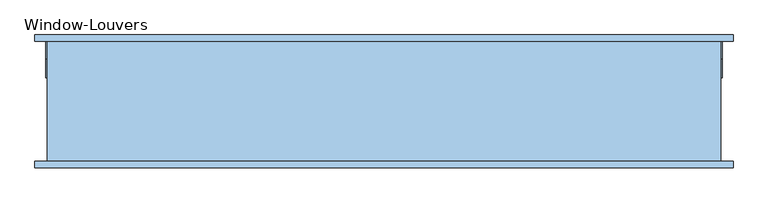
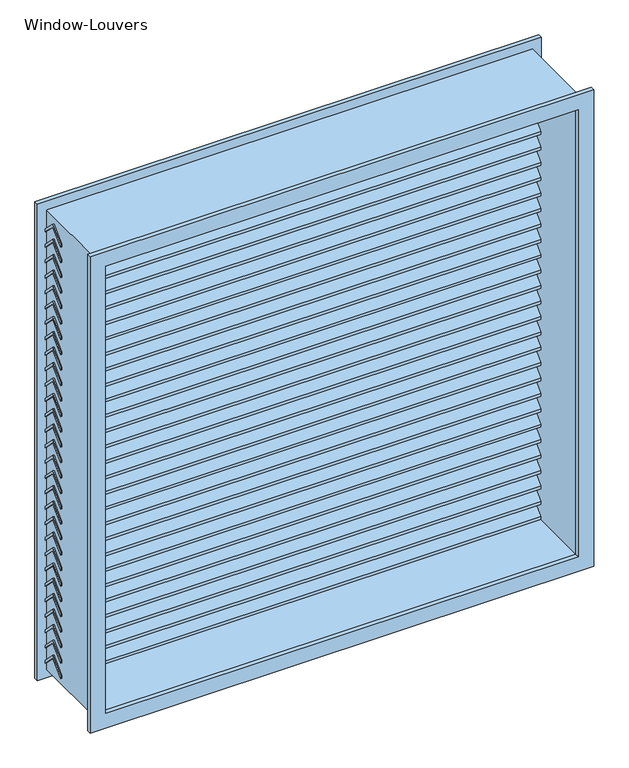
"""IFC4 building model written with IfcOpenShell, lengths in millimetres: window geometry, Window-Louvers : H_WD_AR_B11_Louver_Steel_W1450xH1450."""

from ifc_helpers import new_model, si_unit, frame, origin, place, context, project, spatial, polyline, outline, extrude, source, transform, mapped, element, save


def window_louvers_5883d314(model_context):
    return source(origin(), model_context, "Body", "SweptSolid", [
        extrude(outline(polyline([(118.65, 2234.4100091), (118.65, 2225.429753), (80.55, 2263.529753), (42.45, 2225.429753), (42.45, 2234.4100091), (80.55, 2272.5100091), (118.65, 2234.4100091)])), frame((-702.5, 0.0, 0.0), z_axis=(1.0, 0.0, 0.0), x_axis=(0.0, 1.0, 0.0)), (0.0, 0.0, 1.0), 1405.0),
        extrude(outline(polyline([(118.65, 2187.5200183), (118.65, 2178.5397622), (80.55, 2216.6397622), (42.45, 2178.5397622), (42.45, 2187.5200183), (80.55, 2225.6200183), (118.65, 2187.5200183)])), frame((-702.5, 0.0, 0.0), z_axis=(1.0, 0.0, 0.0), x_axis=(0.0, 1.0, 0.0)), (0.0, 0.0, 1.0), 1405.0),
        extrude(outline(polyline([(118.65, 2140.6300274), (118.65, 2131.6497713), (80.55, 2169.7497713), (42.45, 2131.6497713), (42.45, 2140.6300274), (80.55, 2178.7300274), (118.65, 2140.6300274)])), frame((-702.5, 0.0, 0.0), z_axis=(1.0, 0.0, 0.0), x_axis=(0.0, 1.0, 0.0)), (0.0, 0.0, 1.0), 1405.0),
        extrude(outline(polyline([(118.65, 2093.7400366), (118.65, 2084.7597805), (80.55, 2122.8597805), (42.45, 2084.7597805), (42.45, 2093.7400366), (80.55, 2131.8400366), (118.65, 2093.7400366)])), frame((-702.5, 0.0, 0.0), z_axis=(1.0, 0.0, 0.0), x_axis=(0.0, 1.0, 0.0)), (0.0, 0.0, 1.0), 1405.0),
        extrude(outline(polyline([(118.65, 2046.8500457), (118.65, 2037.8697896), (80.55, 2075.9697896), (42.45, 2037.8697896), (42.45, 2046.8500457), (80.55, 2084.9500457), (118.65, 2046.8500457)])), frame((-702.5, 0.0, 0.0), z_axis=(1.0, 0.0, 0.0), x_axis=(0.0, 1.0, 0.0)), (0.0, 0.0, 1.0), 1405.0),
        extrude(outline(polyline([(118.65, 1999.9600549), (118.65, 1990.9797988), (80.55, 2029.0797988), (42.45, 1990.9797988), (42.45, 1999.9600549), (80.55, 2038.0600549), (118.65, 1999.9600549)])), frame((-702.5, 0.0, 0.0), z_axis=(1.0, 0.0, 0.0), x_axis=(0.0, 1.0, 0.0)), (0.0, 0.0, 1.0), 1405.0),
        extrude(outline(polyline([(118.65, 1953.070064), (118.65, 1944.0898079), (80.55, 1982.1898079), (42.45, 1944.0898079), (42.45, 1953.070064), (80.55, 1991.170064), (118.65, 1953.070064)])), frame((-702.5, 0.0, 0.0), z_axis=(1.0, 0.0, 0.0), x_axis=(0.0, 1.0, 0.0)), (0.0, 0.0, 1.0), 1405.0),
        extrude(outline(polyline([(118.65, 1906.1800732), (118.65, 1897.1998171), (80.55, 1935.2998171), (42.45, 1897.1998171), (42.45, 1906.1800732), (80.55, 1944.2800732), (118.65, 1906.1800732)])), frame((-702.5, 0.0, 0.0), z_axis=(1.0, 0.0, 0.0), x_axis=(0.0, 1.0, 0.0)), (0.0, 0.0, 1.0), 1405.0),
        extrude(outline(polyline([(118.65, 1859.2900823), (118.65, 1850.3098262), (80.55, 1888.4098262), (42.45, 1850.3098262), (42.45, 1859.2900823), (80.55, 1897.3900823), (118.65, 1859.2900823)])), frame((-702.5, 0.0, 0.0), z_axis=(1.0, 0.0, 0.0), x_axis=(0.0, 1.0, 0.0)), (0.0, 0.0, 1.0), 1405.0),
        extrude(outline(polyline([(118.65, 1812.4000915), (118.65, 1803.4198354), (80.55, 1841.5198354), (42.45, 1803.4198354), (42.45, 1812.4000915), (80.55, 1850.5000915), (118.65, 1812.4000915)])), frame((-702.5, 0.0, 0.0), z_axis=(1.0, 0.0, 0.0), x_axis=(0.0, 1.0, 0.0)), (0.0, 0.0, 1.0), 1405.0),
        extrude(outline(polyline([(118.65, 1765.5101006), (118.65, 1756.5298445), (80.55, 1794.6298445), (42.45, 1756.5298445), (42.45, 1765.5101006), (80.55, 1803.6101006), (118.65, 1765.5101006)])), frame((-702.5, 0.0, 0.0), z_axis=(1.0, 0.0, 0.0), x_axis=(0.0, 1.0, 0.0)), (0.0, 0.0, 1.0), 1405.0),
        extrude(outline(polyline([(118.65, 1718.6201098), (118.65, 1709.6398536), (80.55, 1747.7398536), (42.45, 1709.6398536), (42.45, 1718.6201098), (80.55, 1756.7201098), (118.65, 1718.6201098)])), frame((-702.5, 0.0, 0.0), z_axis=(1.0, 0.0, 0.0), x_axis=(0.0, 1.0, 0.0)), (0.0, 0.0, 1.0), 1405.0),
        extrude(outline(polyline([(118.65, 1671.7301189), (118.65, 1662.7498628), (80.55, 1700.8498628), (42.45, 1662.7498628), (42.45, 1671.7301189), (80.55, 1709.8301189), (118.65, 1671.7301189)])), frame((-702.5, 0.0, 0.0), z_axis=(1.0, 0.0, 0.0), x_axis=(0.0, 1.0, 0.0)), (0.0, 0.0, 1.0), 1405.0),
        extrude(outline(polyline([(118.65, 1624.8401281), (118.65, 1615.8598719), (80.55, 1653.9598719), (42.45, 1615.8598719), (42.45, 1624.8401281), (80.55, 1662.9401281), (118.65, 1624.8401281)])), frame((-702.5, 0.0, 0.0), z_axis=(1.0, 0.0, 0.0), x_axis=(0.0, 1.0, 0.0)), (0.0, 0.0, 1.0), 1405.0),
        extrude(outline(polyline([(118.65, 1577.9501372), (118.65, 1568.9698811), (80.55, 1607.0698811), (42.45, 1568.9698811), (42.45, 1577.9501372), (80.55, 1616.0501372), (118.65, 1577.9501372)])), frame((-702.5, 0.0, 0.0), z_axis=(1.0, 0.0, 0.0), x_axis=(0.0, 1.0, 0.0)), (0.0, 0.0, 1.0), 1405.0),
        extrude(outline(polyline([(118.65, 1531.0601464), (118.65, 1522.0798902), (80.55, 1560.1798902), (42.45, 1522.0798902), (42.45, 1531.0601464), (80.55, 1569.1601464), (118.65, 1531.0601464)])), frame((-702.5, 0.0, 0.0), z_axis=(1.0, 0.0, 0.0), x_axis=(0.0, 1.0, 0.0)), (0.0, 0.0, 1.0), 1405.0),
        extrude(outline(polyline([(118.65, 1484.1701555), (118.65, 1475.1898994), (80.55, 1513.2898994), (42.45, 1475.1898994), (42.45, 1484.1701555), (80.55, 1522.2701555), (118.65, 1484.1701555)])), frame((-702.5, 0.0, 0.0), z_axis=(1.0, 0.0, 0.0), x_axis=(0.0, 1.0, 0.0)), (0.0, 0.0, 1.0), 1405.0),
        extrude(outline(polyline([(118.65, 1437.2801646), (118.65, 1428.2999085), (80.55, 1466.3999085), (42.45, 1428.2999085), (42.45, 1437.2801646), (80.55, 1475.3801646), (118.65, 1437.2801646)])), frame((-702.5, 0.0, 0.0), z_axis=(1.0, 0.0, 0.0), x_axis=(0.0, 1.0, 0.0)), (0.0, 0.0, 1.0), 1405.0),
        extrude(outline(polyline([(118.65, 1390.3901738), (118.65, 1381.4099177), (80.55, 1419.5099177), (42.45, 1381.4099177), (42.45, 1390.3901738), (80.55, 1428.4901738), (118.65, 1390.3901738)])), frame((-702.5, 0.0, 0.0), z_axis=(1.0, 0.0, 0.0), x_axis=(0.0, 1.0, 0.0)), (0.0, 0.0, 1.0), 1405.0),
        extrude(outline(polyline([(118.65, 1343.5001829), (118.65, 1334.5199268), (80.55, 1372.6199268), (42.45, 1334.5199268), (42.45, 1343.5001829), (80.55, 1381.6001829), (118.65, 1343.5001829)])), frame((-702.5, 0.0, 0.0), z_axis=(1.0, 0.0, 0.0), x_axis=(0.0, 1.0, 0.0)), (0.0, 0.0, 1.0), 1405.0),
        extrude(outline(polyline([(118.65, 1296.6101921), (118.65, 1287.629936), (80.55, 1325.729936), (42.45, 1287.629936), (42.45, 1296.6101921), (80.55, 1334.7101921), (118.65, 1296.6101921)])), frame((-702.5, 0.0, 0.0), z_axis=(1.0, 0.0, 0.0), x_axis=(0.0, 1.0, 0.0)), (0.0, 0.0, 1.0), 1405.0),
        extrude(outline(polyline([(118.65, 1249.7202012), (118.65, 1240.7399451), (80.55, 1278.8399451), (42.45, 1240.7399451), (42.45, 1249.7202012), (80.55, 1287.8202012), (118.65, 1249.7202012)])), frame((-702.5, 0.0, 0.0), z_axis=(1.0, 0.0, 0.0), x_axis=(0.0, 1.0, 0.0)), (0.0, 0.0, 1.0), 1405.0),
        extrude(outline(polyline([(118.65, 1202.8302104), (118.65, 1193.8499543), (80.55, 1231.9499543), (42.45, 1193.8499543), (42.45, 1202.8302104), (80.55, 1240.9302104), (118.65, 1202.8302104)])), frame((-702.5, 0.0, 0.0), z_axis=(1.0, 0.0, 0.0), x_axis=(0.0, 1.0, 0.0)), (0.0, 0.0, 1.0), 1405.0),
        extrude(outline(polyline([(118.65, 1155.9402195), (118.65, 1146.9599634), (80.55, 1185.0599634), (42.45, 1146.9599634), (42.45, 1155.9402195), (80.55, 1194.0402195), (118.65, 1155.9402195)])), frame((-702.5, 0.0, 0.0), z_axis=(1.0, 0.0, 0.0), x_axis=(0.0, 1.0, 0.0)), (0.0, 0.0, 1.0), 1405.0),
        extrude(outline(polyline([(118.65, 1109.0502287), (118.65, 1100.0699726), (80.55, 1138.1699726), (42.45, 1100.0699726), (42.45, 1109.0502287), (80.55, 1147.1502287), (118.65, 1109.0502287)])), frame((-702.5, 0.0, 0.0), z_axis=(1.0, 0.0, 0.0), x_axis=(0.0, 1.0, 0.0)), (0.0, 0.0, 1.0), 1405.0),
        extrude(outline(polyline([(118.65, 1062.1602378), (118.65, 1053.1799817), (80.55, 1091.2799817), (42.45, 1053.1799817), (42.45, 1062.1602378), (80.55, 1100.2602378), (118.65, 1062.1602378)])), frame((-702.5, 0.0, 0.0), z_axis=(1.0, 0.0, 0.0), x_axis=(0.0, 1.0, 0.0)), (0.0, 0.0, 1.0), 1405.0),
        extrude(outline(polyline([(118.65, 1015.270247), (118.65, 1006.2899909), (80.55, 1044.3899909), (42.45, 1006.2899909), (42.45, 1015.270247), (80.55, 1053.370247), (118.65, 1015.270247)])), frame((-702.5, 0.0, 0.0), z_axis=(1.0, 0.0, 0.0), x_axis=(0.0, 1.0, 0.0)), (0.0, 0.0, 1.0), 1405.0),
        extrude(outline(polyline([(118.65, 2281.3), (118.65, 2272.3197439), (80.55, 2310.4197439), (42.45, 2272.3197439), (42.45, 2281.3), (80.55, 2319.4), (118.65, 2281.3)])), frame((-702.5, 0.0, 0.0), z_axis=(1.0, 0.0, 0.0), x_axis=(0.0, 1.0, 0.0)), (0.0, 0.0, 1.0), 1405.0),
        extrude(outline(polyline([(118.65, 968.3802561), (118.65, 959.4), (80.55, 997.5), (42.45, 959.4), (42.45, 968.3802561), (80.55, 1006.4802561), (118.65, 968.3802561)])), frame((-702.5, 0.0, 0.0), z_axis=(1.0, 0.0, 0.0), x_axis=(0.0, 1.0, 0.0)), (0.0, 0.0, 1.0), 1405.0),
        extrude(outline(polyline([(2364.4, -725.0), (914.4, -725.0), (914.4, 725.0), (2364.4, 725.0), (2364.4, -725.0)]), holes=[polyline([(2319.4, -680.0), (2319.4, 680.0), (959.4, 680.0), (959.4, -680.0), (2319.4, -680.0)])]), frame((0.0, 118.65, 0.0), z_axis=(0.0, 1.0, 0.0), x_axis=(0.0, 0.0, 1.0)), (0.0, 0.0, 1.0), 12.7),
        extrude(outline(polyline([(2364.4, 725.0), (2364.4, -725.0), (914.4, -725.0), (914.4, 725.0), (2364.4, 725.0)]), holes=[polyline([(2319.4, 680.0), (959.4, 680.0), (959.4, -680.0), (2319.4, -680.0), (2319.4, 680.0)])]), frame((0.0, -144.05, 0.0), z_axis=(0.0, 1.0, 0.0), x_axis=(0.0, 0.0, 1.0)), (0.0, 0.0, 1.0), 12.7),
        extrude(outline(polyline([(2338.45, 699.05), (2338.45, -699.05), (940.35, -699.05), (940.35, 699.05), (2338.45, 699.05)]), holes=[polyline([(2319.4, 680.0), (959.4, 680.0), (959.4, -680.0), (2319.4, -680.0), (2319.4, 680.0)])]), frame((0.0, -131.35, 0.0), z_axis=(0.0, 1.0, 0.0), x_axis=(0.0, 0.0, 1.0)), (0.0, 0.0, 1.0), 250.0),
    ])


if __name__ == "__main__":
    model = new_model("IFC4")
    model_context = context("Model", 3, world=origin())
    ifc_project = project(units=[si_unit("LENGTHUNIT", "METRE", prefix="MILLI")], contexts=[model_context])
    site = spatial("IfcSite", under=ifc_project)
    building = spatial("IfcBuilding", under=site)
    placement = place(None, origin())
    window_louvers_shape = window_louvers_5883d314(model_context)
    element("IfcWindow", 1, ObjectType="Window-Louvers : H_WD_AR_B11_Louver_Steel_W1450xH1450", at=placement, inside=building, context=model_context, shape_type="MappedRepresentation", body=[
        mapped(window_louvers_shape, transform((0.0, 0.0, 0.0), x_axis=(1.0, 0.0, 0.0), y_axis=(0.0, 1.0, 0.0), z_axis=(0.0, 0.0, 1.0))),
    ])
    save(model, "model.ifc")

# Revit data of these elements
# Type "Window-Louvers : H_WD_AR_B11_Louver_Steel_W1450xH1450"
#   Type Mark = "286"
#   Assembly Code = "B20"
#   Visual Light Transmittance = 0.9
#   Solar Heat Gain Coefficient = 0.78
#   Max Height = 1450.508 mm
#   Height = 1450 mm
#   Heat Transfer Coefficient (U) = 3.6886 W/(m²·K)
#   Blade Width [instance default] = 1405 mm
#   Blade Vertical Thickness = 8.98 mm
#   Blade Thickness = 6.35 mm
#   Blade Spacing = 38.1 mm
#   Blade Height = 47.08 mm
#   Blade Depth = 76.2 mm
#   Blade Angle = 45.00°
#   Default Sill Height = 914.4 mm
#   Trim Projection_Exterior = 12.7 mm
#   Trim Projection_Interior = 12.7 mm
#   Trim Width_Exterior = 45 mm
#   Trim Width_Interior = 45 mm
#   Width = 1450 mm
#   Max Blade Count = 30
#   Define Thermal Properties by = 1
#   Blade Count = 29
#   Frame Material = Birch
#   Louver Material = Birch
#   Trim Exterior Material = Birch
#   Trim Interior Material = Birch
#   Thermal Resistance (R) = 0
#   Construction Type Id = ""
#   Wall Closure = (empty or 0)
#   Analytic Construction = (empty or 0)
# Element 1 (IfcWindow, "Window-Louvers : H_WD_AR_B11_Louver_Steel_W1450xH1450")
#   Materials on its faces: "00_Metal_Steel"
# Materials
#   "Birch": class "Wood", colour RGB 224 178 126, transparency 0, Description = "Betula Alleghaniensis", Cost = 0
#   "00_Metal_Steel": class "Metal", colour RGB 148 148 148, transparency 0, Description = "Steel", Cost = 0, Image = Doors - Windows.Glazed Curtain Walls.Stainless Steel Curtain Wall.jpg
